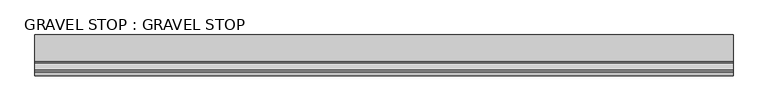
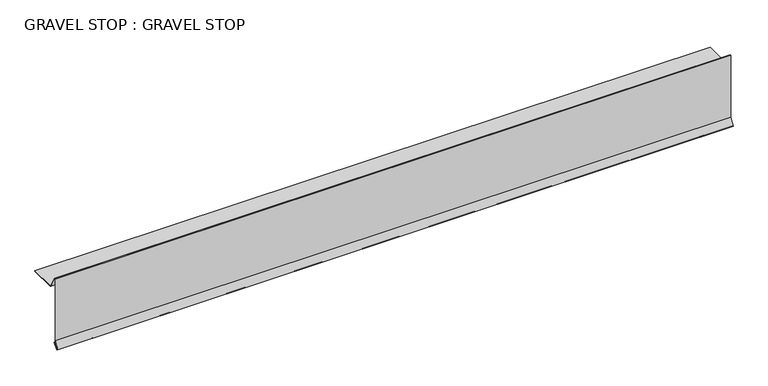
"""IFC4 building model written with IfcOpenShell, lengths in millimetres: proxy geometry, GRAVEL STOP : GRAVEL STOP."""

from ifc_helpers import new_model, si_unit, frame, origin, place, context, project, spatial, polyline, outline, extrude, source, transform, mapped, element, save


def gravel_stop_gravel_stop_d8bdad0e(model_context):
    return source(origin(), model_context, "Body", "SweptSolid", [
        extrude(outline(polyline([(-5587.6106629, 40061.0736754), (-5591.684607, 40064.1815506), (-5580.0356381, 40085.5191254), (-5580.0356381, 40278.1940248), (-5577.0037237, 40279.0064238), (-5556.3332702, 40243.204148), (-5552.58096, 40241.0377507), (-5475.1230533, 40241.0377507), (-5475.1230533, 40239.6266397), (-5552.959066, 40239.6266397), (-5557.3662751, 40242.1711431), (-5577.6843899, 40277.3631503), (-5578.6245271, 40277.1112413), (-5578.6245271, 40085.1590213), (-5589.8655469, 40064.5686925), (-5587.7358967, 40062.9440538), (-5574.2139721, 40076.4659785), (-5573.2161659, 40075.4681723), (-5587.6106629, 40061.0736754)])), frame((12382.7678845, 0.0, 0.0), z_axis=(1.0, 0.0, 0.0), x_axis=(0.0, 1.0, 0.0)), (0.0, 0.0, 1.0), 2000.25),
    ])


if __name__ == "__main__":
    model = new_model("IFC4")
    model_context = context("Model", 3, world=origin())
    ifc_project = project(units=[si_unit("LENGTHUNIT", "METRE", prefix="MILLI")], contexts=[model_context])
    site = spatial("IfcSite", under=ifc_project)
    building = spatial("IfcBuilding", under=site)
    placement = place(None, origin())
    gravel_stop_gravel_stop_shape = gravel_stop_gravel_stop_d8bdad0e(model_context)
    element("IfcBuildingElementProxy", 1, Name="GRAVEL STOP : GRAVEL STOP", ObjectType="GRAVEL STOP : GRAVEL STOP", at=placement, inside=building, context=model_context, shape_type="MappedRepresentation", body=[
        mapped(gravel_stop_gravel_stop_shape, transform((0.0, 0.0, 0.0), x_axis=(1.0, 0.0, 0.0), y_axis=(0.0, 1.0, 0.0), z_axis=(0.0, 0.0, 1.0))),
    ])
    save(model, "model.ifc")

# Revit data of these elements
# Type "GRAVEL STOP : GRAVEL STOP"
#   NameOverride = "GRAVEL STOP"
# Element 1 (IfcBuildingElementProxy, "GRAVEL STOP : GRAVEL STOP")
#   Materials on its faces: "GRAVEL STOP REQUIRED WITH GRAVEL SURFACE SYSTEMS"
# Materials
#   "GRAVEL STOP REQUIRED WITH GRAVEL SURFACE SYSTEMS": class "Unassigned", colour RGB 170 170 127, transparency 0
